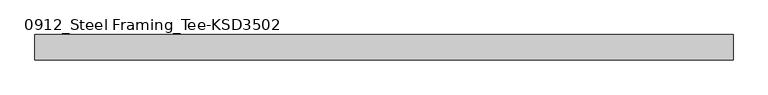
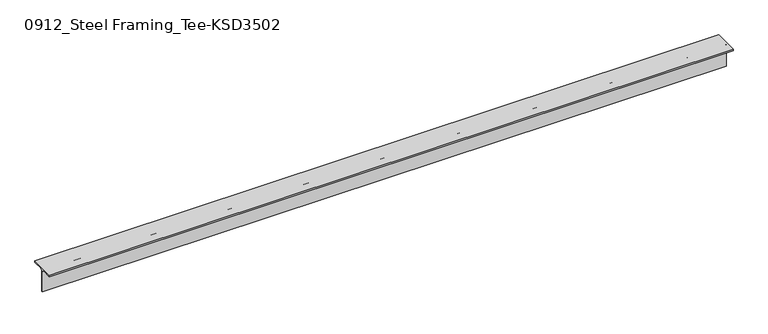
"""IFC4 building model written with IfcOpenShell, lengths in millimetres: member geometry, 0912_Steel Framing_Tee-KSD3502 : H_SB_ASB_CT-150x150x6.5x9."""

from ifc_helpers import new_model, si_unit, point, frame, frame_2d, origin, place, context, project, spatial, polyline, circle_curve, trimmed, segment, composite_curve, outline, extrude, source, transform, mapped, element, save


def member_0912_steel_framing_tee_ksd3502_21fe7dae(model_context):
    return source(origin(), model_context, "Body", "SweptSolid", [
        extrude(outline(composite_curve([segment(polyline([(75.0, 75.0), (75.0, 66.0), (16.25, 66.0)]), True, "CONTINUOUS"), segment(trimmed(circle_curve(frame_2d((16.25, 53.0)), 13.0), [point((16.25, 66.0))], [point((3.25, 53.0))], True, "CARTESIAN"), True, "CONTINUOUS"), segment(polyline([(3.25, 53.0), (3.25, -75.0), (-3.25, -75.0), (-3.25, 53.0)]), True, "CONTINUOUS"), segment(trimmed(circle_curve(frame_2d((-16.25, 53.0)), 13.0), [point((-3.25, 53.0))], [point((-16.25, 66.0))], True, "CARTESIAN"), True, "CONTINUOUS"), segment(polyline([(-16.25, 66.0), (-75.0, 66.0), (-75.0, 75.0), (75.0, 75.0)]), True, "CONTINUOUS")], self_intersect=False)), frame((-2059.5, 0.0, 0.0), z_axis=(1.0, 0.0, 0.0), x_axis=(0.0, 1.0, 0.0)), (0.0, 0.0, 1.0), 4105.6),
    ])


if __name__ == "__main__":
    model = new_model("IFC4")
    model_context = context("Model", 3, world=origin())
    ifc_project = project(units=[si_unit("LENGTHUNIT", "METRE", prefix="MILLI")], contexts=[model_context])
    site = spatial("IfcSite", under=ifc_project)
    building = spatial("IfcBuilding", under=site)
    placement = place(None, origin())
    member_0912_steel_framing_tee_ksd3502_shape = member_0912_steel_framing_tee_ksd3502_21fe7dae(model_context)
    element("IfcMember", 1, ObjectType="0912_Steel Framing_Tee-KSD3502 : H_SB_ASB_CT-150x150x6.5x9", at=placement, inside=building, context=model_context, shape_type="MappedRepresentation", body=[
        mapped(member_0912_steel_framing_tee_ksd3502_shape, transform((0.0, 0.0, 0.0), x_axis=(1.0, 0.0, 0.0), y_axis=(0.0, 1.0, 0.0), z_axis=(0.0, 0.0, 1.0))),
    ])
    save(model, "model.ifc")

# Revit data of these elements
# Type "0912_Steel Framing_Tee-KSD3502 : H_SB_ASB_CT-150x150x6.5x9"
#   H_WM Code_1 = "S01AA003-00001 | Main Steel Structure Fabrication Work | Shelter/Building | Light Steel - Standard (30KG/M>Weight) | Material: (   )"
#   H_WM Code_2 = "S03AA029-00001 | Main Steel Structure Erection Work | Shelter/Building | Light Steel (30KG/M>Weight) | Material: (   )"
#   H_WM Code_3 = "S01AA010-00001 | Main Steel Structure Fabrication Work | Shelter/Building | Steel Painting/Coating | for Non-Fireproofed Steel Surface, Surface Preparation, Primer, Second & Final Coat | Material: (   )"
#   H_Q'ty Cal Type Tag = "SB-Q2"
#   Width = 15.0 cm
#   Web Thickness = 0.65 cm
#   Web Fillet = 1.3 cm
#   Section Area = 23.39 cm²
#   Perimeter = 0.60 m²/m
#   Nominal Weight = 18.40 kgf/m
#   Height = 15.0 cm
#   Flange Thickness = 0.9 cm
#   Centroid Vertical = 7.5 cm
#   Centroid Horizontal = 7.5 cm
#   Length [instance default] = 1.5000 m
#   Structural Material [instance default] = Steel, 45-345
#   Warping Constant = (empty or 0)
#   Torsional Moment of Inertia = 0
#   Section Name Key = ""
#   Plastic Modulus weak axis = 0
#   Plastic Modulus strong axis = 0
#   Moment of Inertia weak axis = 0
#   Moment of Inertia strong axis = 0
#   Elastic Modulus weak axis = 0
#   Elastic Modulus strong axis = 0
#   Bolt Spacing = 0
#   Assembly Code = ""
# Element 1 (IfcMember, "0912_Steel Framing_Tee-KSD3502 : H_SB_ASB_CT-150x150x6.5x9")
#   Structural Material = none
# Materials
#   "Steel, 45-345": class "Metal", colour RGB 189 187 185, transparency 0, Description = "Steel 345 MPa", Cost = 0
